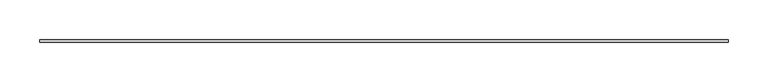
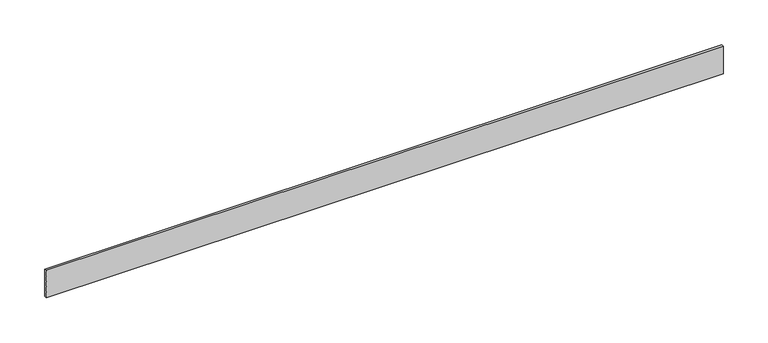
"""IFC4 building model written with IfcOpenShell, lengths in millimetres: proxy geometry, Generic Models 3:Generic Models 1:3:Generic Models 1:3 : Generic Models 3:Generic Models 1:300625:336034:Generic Models 1:3:Generic Models 1:3 : Generic Models 3:Generic Models 1:300625:336034 : Generic Models 3:Generic Models 1:3:Generic Models 1:3 : Generic Models 3:Generic Models 1:300625:336034:6 : Generic Models 3:Generic Models 1:3:Generic Models 1:3 : Generic Models 3:Generic Models 1:300625:336034:Generic Models 1:3:Generic Models 1:3 : Generic Models 3:Generic Models 1:300625:336034 : Generic Models 3:Generic Models 1:3:Generic Models 1:3 : Generic Models 3:Generic Models 1:300625:336034:301191."""

import ifcopenshell
import ifcopenshell.guid

model = None  # the IFC model being written
_history = None  # IfcOwnerHistory: only IFC2X3 demands one
_inside = {}  # id of a spatial element -> (the spatial element, [elements in it])
_under = {}  # id of a project, library or spatial element -> (it, [spatial elements below it])
_declared = {}  # id of a project -> (the project, [libraries it declares])
_typed = {}  # id of a type object -> (the type object, [elements of that type])
_made_of = {}  # id of a material, layer set ... -> (it, [elements and type objects made of it])


def new_model(schema):
    """Start an empty IFC model of exactly this schema.

    Asked for "IFC4X3", IfcOpenShell would pick the latest addendum, in which some entities
    have other attributes; the version numbers below select the first issue.
    IFC2X3 requires an IfcOwnerHistory on every rooted entity: one is made here for all.
    """
    global model, _history
    if schema == "IFC4X3":
        model = ifcopenshell.file(schema_version=(4, 3, 0, 0))
    else:
        model = ifcopenshell.file(schema=schema)
    _inside.clear()
    _under.clear()
    _declared.clear()
    _typed.clear()
    _made_of.clear()
    _history = None
    if model.schema == "IFC2X3":
        org = make("IfcOrganization", Name="unknown")
        user = make(
            "IfcPersonAndOrganization",
            ThePerson=make("IfcPerson", FamilyName="unknown"),
            TheOrganization=org,
        )
        app = make(
            "IfcApplication",
            ApplicationDeveloper=org,
            Version="unknown",
            ApplicationFullName="unknown",
            ApplicationIdentifier="unknown",
        )
        _history = make(
            "IfcOwnerHistory",
            OwningUser=user,
            OwningApplication=app,
            ChangeAction="ADDED",
            CreationDate=0,
        )
    return model


def make(cls, **values):
    """One entity of the class cls with the attributes given. An attribute that is None is left unset."""
    return model.create_entity(
        cls, **{name: value for name, value in values.items() if value is not None}
    )


def rooted(cls, **values):
    """An entity with a GlobalId (a new one), such as an element, a storey or a relation."""
    return make(cls, GlobalId=ifcopenshell.guid.new(), OwnerHistory=_history, **values)


def si_unit(unit_type, name, prefix=None):
    """IfcSIUnit, for example si_unit("LENGTHUNIT", "METRE", prefix="MILLI")."""
    return make("IfcSIUnit", UnitType=unit_type, Prefix=prefix, Name=name)


def assignment(units):
    """IfcUnitAssignment: the units of a project."""
    return None if units is None else make("IfcUnitAssignment", Units=units)


def point(xyz):
    """IfcCartesianPoint."""
    return None if xyz is None else make("IfcCartesianPoint", Coordinates=xyz)


def direction(xyz):
    """IfcDirection."""
    return None if xyz is None else make("IfcDirection", DirectionRatios=xyz)


def frame(location, z_axis=None, x_axis=None):
    """IfcAxis2Placement3D, a coordinate frame: its origin and axes. An axis left out is left unset."""
    return make(
        "IfcAxis2Placement3D",
        Location=point(location),
        Axis=direction(z_axis),
        RefDirection=direction(x_axis),
    )


def origin():
    """The frame at (0, 0, 0) with its axes left unset."""
    return frame((0.0, 0.0, 0.0))


def place(relative_to, where):
    """IfcLocalPlacement: puts the frame where relative to a parent placement (None: the world)."""
    return make(
        "IfcLocalPlacement", PlacementRelTo=relative_to, RelativePlacement=where
    )


def context(
    kind, dimensions, precision=None, world=None, true_north=None, identifier=None
):
    """IfcGeometricRepresentationContext, for example the 3D "Model" context."""
    return make(
        "IfcGeometricRepresentationContext",
        ContextIdentifier=identifier,
        ContextType=kind,
        CoordinateSpaceDimension=dimensions,
        Precision=precision,
        WorldCoordinateSystem=world,
        TrueNorth=true_north,
    )


def project(units=None, contexts=None):
    """IfcProject with its units and contexts."""
    return rooted(
        "IfcProject",
        Name="project",
        RepresentationContexts=contexts,
        UnitsInContext=assignment(units),
    )


def spatial(cls, under=None, at=None, **own):
    """A site, building, storey or space (cls), placed at a placement, below another one or the project."""
    s = rooted(cls, ObjectPlacement=at, **own)
    if under is not None:
        _under.setdefault(under.id(), (under, []))[1].append(s)
    return s


def polyline(points):
    """IfcPolyline through the points."""
    return make("IfcPolyline", Points=[point(p) for p in points])


def outline(outer, holes=None, kind="AREA"):
    """IfcArbitraryClosedProfileDef: a profile drawn as a closed curve; with holes, ...WithVoids."""
    if holes is None:
        return make("IfcArbitraryClosedProfileDef", ProfileType=kind, OuterCurve=outer)
    return make(
        "IfcArbitraryProfileDefWithVoids",
        ProfileType=kind,
        OuterCurve=outer,
        InnerCurves=holes,
    )


def extrude(swept, where, along, depth):
    """IfcExtrudedAreaSolid: the profile swept, set in the frame where, extruded along a direction by depth."""
    return make(
        "IfcExtrudedAreaSolid",
        SweptArea=swept,
        Position=where,
        ExtrudedDirection=direction(along),
        Depth=depth,
    )


def shape(context_of_items, identifier, shape_type, items):
    """IfcShapeRepresentation: the items that make up one representation, for example the "Body"."""
    return make(
        "IfcShapeRepresentation",
        ContextOfItems=context_of_items,
        RepresentationIdentifier=identifier,
        RepresentationType=shape_type,
        Items=items,
    )


def source(mapping_origin, context_of_items, identifier, shape_type, items):
    """IfcRepresentationMap: a shape defined once, which mapped items show again and again."""
    return make(
        "IfcRepresentationMap",
        MappingOrigin=mapping_origin,
        MappedRepresentation=shape(context_of_items, identifier, shape_type, items),
    )


def transform(
    local_origin,
    x_axis=None,
    y_axis=None,
    z_axis=None,
    scale=None,
    scale2=None,
    scale3=None,
    uniform=True,
):
    """IfcCartesianTransformationOperator3D, or its non-uniform kind. x_axis, y_axis, z_axis: its Axis1, 2, 3."""
    if uniform:
        return make(
            "IfcCartesianTransformationOperator3D",
            Axis1=direction(x_axis),
            Axis2=direction(y_axis),
            LocalOrigin=point(local_origin),
            Scale=scale,
            Axis3=direction(z_axis),
        )
    return make(
        "IfcCartesianTransformationOperator3DnonUniform",
        Axis1=direction(x_axis),
        Axis2=direction(y_axis),
        LocalOrigin=point(local_origin),
        Scale=scale,
        Axis3=direction(z_axis),
        Scale2=scale2,
        Scale3=scale3,
    )


def mapped(mapping_source, mapping_target):
    """IfcMappedItem: shows the shape of a source again, moved by a transform."""
    return make(
        "IfcMappedItem", MappingSource=mapping_source, MappingTarget=mapping_target
    )


def made_of(thing, what):
    """Note that an element or type object is made of a material, layer set ...; save() writes the relation."""
    if what is not None:
        _made_of.setdefault(what.id(), (what, []))[1].append(thing)
    return thing


def element(
    cls,
    number,
    at=None,
    inside=None,
    cuts=None,
    type_object=None,
    material=None,
    context=None,
    identifier="Body",
    shape_type=None,
    held_by="IfcProductDefinitionShape",
    body=None,
    shapes=None,
    **own,
):
    """One element of the class cls, such as IfcWall. Its Tag is "e" and its number.

    at: its placement. inside: the storey or other place that contains it. cuts: it is an
    opening in that element (IfcRelVoidsElement). A single representation is given by context,
    identifier, shape_type and body (its items); several are given by shapes. held_by: the class
    of the entity that holds the representations. save() writes the other relations.
    """
    e = rooted(cls, Tag="e%d" % number, ObjectPlacement=at, **own)
    if body is not None:
        shapes = [shape(context, identifier, shape_type, body)]
    if shapes is not None:
        e.Representation = make(held_by, Representations=shapes)
    if inside is not None:
        _inside.setdefault(inside.id(), (inside, []))[1].append(e)
    if cuts is not None:
        rooted(
            "IfcRelVoidsElement", RelatingBuildingElement=cuts, RelatedOpeningElement=e
        )
    if type_object is not None:
        _typed.setdefault(type_object.id(), (type_object, []))[1].append(e)
    return made_of(e, material)


def aggregate(whole, parts):
    """IfcRelAggregates: a whole, such as a stair, and the parts it consists of."""
    return rooted("IfcRelAggregates", RelatingObject=whole, RelatedObjects=parts)


def save(model, path):
    """Write the relations noted so far, then the file.

    IfcRelAggregates (storeys below a building ...), IfcRelContainedInSpatialStructure (elements
    in a storey), IfcRelDefinesByType, IfcRelAssociatesMaterial and IfcRelDeclares: one each for
    every whole, place, type object, material and project.
    """
    for whole, parts in _under.values():
        aggregate(whole, parts)
    for where, things in _inside.values():
        rooted(
            "IfcRelContainedInSpatialStructure",
            RelatedElements=things,
            RelatingStructure=where,
        )
    for kind, things in _typed.values():
        rooted("IfcRelDefinesByType", RelatedObjects=things, RelatingType=kind)
    for what, things in _made_of.values():
        rooted("IfcRelAssociatesMaterial", RelatedObjects=things, RelatingMaterial=what)
    for by, libraries in _declared.values():
        rooted("IfcRelDeclares", RelatingContext=by, RelatedDefinitions=libraries)
    model.write(path)


def generic_models_5c589dd8(model_context):
    return source(origin(), model_context, "Body", "SweptSolid", [
        extrude(outline(polyline([(593680.9367239, -579000.6913841), (593680.9367239, -579003.8663841), (592812.5742239, -579003.8663841), (592812.5742239, -579000.6913841), (593680.9367239, -579000.6913841)])), frame((0.0, 0.0, 2447.925), z_axis=(0.0, 0.0, 1.0), x_axis=(1.0, 0.0, 0.0)), (0.0, 0.0, 1.0), 36.9653358),
    ])


if __name__ == "__main__":
    model = new_model("IFC4")
    model_context = context("Model", 3, world=origin())
    ifc_project = project(units=[si_unit("LENGTHUNIT", "METRE", prefix="MILLI")], contexts=[model_context])
    site = spatial("IfcSite", under=ifc_project)
    building = spatial("IfcBuilding", under=site)
    placement = place(None, origin())
    generic_models_shape = generic_models_5c589dd8(model_context)
    element("IfcBuildingElementProxy", 1, Name="Generic Models 3:Generic Models 1:3:Generic Models 1:3 : Generic Models 3:Generic Models 1:300625:336034:Generic Models 1:3:Generic Models 1:3 : Generic Models 3:Generic Models 1:300625:336034 : Generic Models 3:Generic Models 1:3:Generic Models 1:3 : Generic Models 3:Generic Models 1:300625:336034:6 : Generic Models 3:Generic Models 1:3:Generic Models 1:3 : Generic Models 3:Generic Models 1:300625:336034:Generic Models 1:3:Generic Models 1:3 : Generic Models 3:Generic Models 1:300625:336034 : Generic Models 3:Generic Models 1:3:Generic Models 1:3 : Generic Models 3:Generic Models 1:300625:336034:301191", ObjectType="Generic Models 3:Generic Models 1:3:Generic Models 1:3 : Generic Models 3:Generic Models 1:300625:336034:Generic Models 1:3:Generic Models 1:3 : Generic Models 3:Generic Models 1:300625:336034 : Generic Models 3:Generic Models 1:3:Generic Models 1:3 : Generic Models 3:Generic Models 1:300625:336034:6 : Generic Models 3:Generic Models 1:3:Generic Models 1:3 : Generic Models 3:Generic Models 1:300625:336034:Generic Models 1:3:Generic Models 1:3 : Generic Models 3:Generic Models 1:300625:336034 : Generic Models 3:Generic Models 1:3:Generic Models 1:3 : Generic Models 3:Generic Models 1:300625:336034:301191", at=placement, inside=building, context=model_context, shape_type="MappedRepresentation", body=[
        mapped(generic_models_shape, transform((0.0, 0.0, 0.0), x_axis=(1.0, 0.0, 0.0), y_axis=(0.0, 1.0, 0.0), z_axis=(0.0, 0.0, 1.0))),
    ])
    save(model, "model.ifc")

# Revit data of these elements
# Type "Generic Models 3:Generic Models 1:3:Generic Models 1:3 : Generic Models 3:Generic Models 1:300625:336034:Generic Models 1:3:Generic Models 1:3 : Generic Models 3:Generic Models 1:300625:336034 : Generic Models 3:Generic Models 1:3:Generic Models 1:3 : Generic Models 3:Generic Models 1:300625:336034:6 : Generic Models 3:Generic Models 1:3:Generic Models 1:3 : Generic Models 3:Generic Models 1:300625:336034:Generic Models 1:3:Generic Models 1:3 : Generic Models 3:Generic Models 1:300625:336034 : Generic Models 3:Generic Models 1:3:Generic Models 1:3 : Generic Models 3:Generic Models 1:300625:336034:301191"
#   NameOverride = "Generic Models 3:Generic Models 1:3:Generic Models 1:3 : Generic Models 3:Generic Models 1:300625:336034:Generic Models 1:3:Generic Models 1:3 : Generic Models 3:Generic Models 1:300625:336034 : Generic Models 3:Generic Models 1:3:Generic Models 1:3 : Generic Models 3:Generic Models 1:300625:336034:301191"
#   ObjectTypeOverride = "Generic Models 1:3:Generic Models 1:3 : Generic Models 3:Generic Models 1:300625:336034 : Generic Models 3:Generic Models 1:3:Generic Models 1:3 : Generic Models 3:Generic Models 1:300625:336034"
#   Reference = "Generic Models 1"
#   Tag = "301191"
# Element 1 (IfcBuildingElementProxy, "Generic Models 3:Generic Models 1:3:Generic Models 1:3 : Generic Models 3:Generic Models 1:300625:336034:Generic Models 1:3:Generic Models 1:3 : Generic Models 3:Generic Models 1:300625:336034 : Generic Models 3:Generic Models 1:3:Generic Models 1:3 : Generic Models 3:Generic Models 1:300625:336034:6 : Generic Models 3:Generic Models 1:3:Generic Models 1:3 : Generic Models 3:Generic Models 1:300625:336034:Generic Models 1:3:Generic Models 1:3 : Generic Models 3:Generic Models 1:300625:336034 : Generic Models 3:Generic Models 1:3:Generic Models 1:3 : Generic Models 3:Generic Models 1:300625:336034:301191")
#   Materials on its faces: "COMPRESSIBE THERMAL GASKET SANDWICHED BETWEEN METAL COMPONENTS"
# Materials
#   "COMPRESSIBE THERMAL GASKET SANDWICHED BETWEEN METAL COMPONENTS": class "Unassigned", colour RGB 58 208 21, transparency 0, Cost = 0
